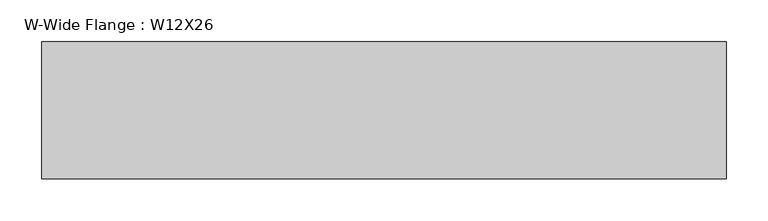
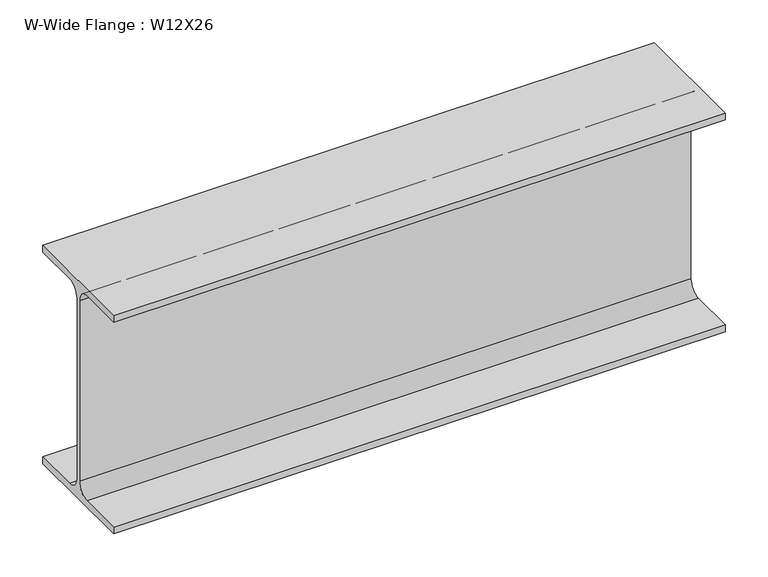
"""IFC4 building model written with IfcOpenShell, lengths in millimetres: beam geometry, W-Wide Flange : W12X26."""

from ifc_helpers import new_model, si_unit, point, frame, frame_2d, origin, place, context, project, spatial, polyline, circle_curve, trimmed, segment, composite_curve, outline, extrude, source, transform, mapped, element, save


def w_wide_flange_w12x26_7fa1df94(model_context):
    return source(origin(), model_context, "Body", "SweptSolid", [
        extrude(outline(composite_curve([segment(polyline([(-82.4011719, -145.5539063), (-20.2902344, -145.5539063)]), True, "CONTINUOUS"), segment(trimmed(circle_curve(frame_2d((-20.2902344, -128.190625)), 17.3632812), [point((-20.2902344, -145.5539063))], [point((-2.9269531, -128.190625))], True, "CARTESIAN"), True, "CONTINUOUS"), segment(polyline([(-2.9269531, -128.190625), (-2.9269531, 128.190625)]), True, "CONTINUOUS"), segment(trimmed(circle_curve(frame_2d((-20.2902344, 128.190625)), 17.3632812), [point((-2.9269531, 128.190625))], [point((-20.2902344, 145.5539062))], True, "CARTESIAN"), True, "CONTINUOUS"), segment(polyline([(-20.2902344, 145.5539062), (-82.4011719, 145.5539062), (-82.4011719, 155.178125), (82.4011719, 155.178125), (82.4011719, 145.5539062), (20.2902344, 145.5539062)]), True, "CONTINUOUS"), segment(trimmed(circle_curve(frame_2d((20.2902344, 128.190625)), 17.3632812), [point((20.2902344, 145.5539062))], [point((2.9269531, 128.190625))], True, "CARTESIAN"), True, "CONTINUOUS"), segment(polyline([(2.9269531, 128.190625), (2.9269531, -128.190625)]), True, "CONTINUOUS"), segment(trimmed(circle_curve(frame_2d((20.2902344, -128.190625)), 17.3632812), [point((2.9269531, -128.190625))], [point((20.2902344, -145.5539063))], True, "CARTESIAN"), True, "CONTINUOUS"), segment(polyline([(20.2902344, -145.5539063), (82.4011719, -145.5539063), (82.4011719, -155.178125), (-82.4011719, -155.178125), (-82.4011719, -145.5539063)]), True, "CONTINUOUS")], self_intersect=False)), frame((-282.575, 0.0, 0.0), z_axis=(1.0, 0.0, 0.0), x_axis=(0.0, 1.0, 0.0)), (0.0, 0.0, 1.0), 822.1761719),
    ])


if __name__ == "__main__":
    model = new_model("IFC4")
    model_context = context("Model", 3, world=origin())
    ifc_project = project(units=[si_unit("LENGTHUNIT", "METRE", prefix="MILLI")], contexts=[model_context])
    site = spatial("IfcSite", under=ifc_project)
    building = spatial("IfcBuilding", under=site)
    placement = place(None, origin())
    w_wide_flange_w12x26_shape = w_wide_flange_w12x26_7fa1df94(model_context)
    element("IfcBeam", 1, ObjectType="W-Wide Flange : W12X26", at=placement, inside=building, context=model_context, shape_type="MappedRepresentation", body=[
        mapped(w_wide_flange_w12x26_shape, transform((0.0, 0.0, 0.0), x_axis=(1.0, 0.0, 0.0), y_axis=(0.0, 1.0, 0.0), z_axis=(0.0, 0.0, 1.0))),
    ])
    save(model, "model.ifc")

# Revit data of these elements
# Type "W-Wide Flange : W12X26"
#   Assembly Code = "B10"
#   W = 26
#   Start Extension Calculation [instance default] = 10' - 0"
#   Start Extension [instance default] = -0' - 0 1/2"
#   End Extension Calculation [instance default] = 10' - 0"
#   End Extension [instance default] = -0' - 0 1/2"
#   Length [instance default] = 5' - 0"
#   bf = 0' - 6 125/256"
#   d = 1' - 0 7/32"
#   k = 0' - 1 1/16"
#   k2 = 0' - 0 175/256"
#   tf = 0' - 0 97/256"
#   tw = 0' - 0 59/256"
#   A = 0.05 SF
#   Beam Material [instance default] = Metal - Steel - ASTM A992
# Element 1 (IfcBeam, "W-Wide Flange : W12X26")
#   Materials on its faces: "Metal - Steel - ASTM A992"
# Materials
#   "Metal - Steel - ASTM A992": class "Metal", colour RGB 128 0 0, transparency 0
